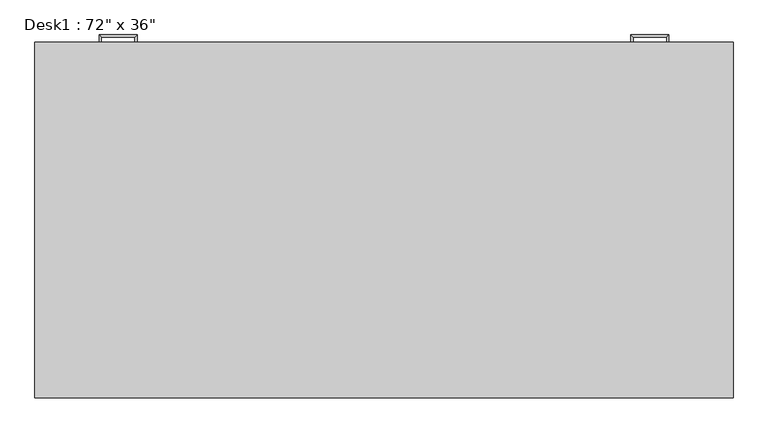
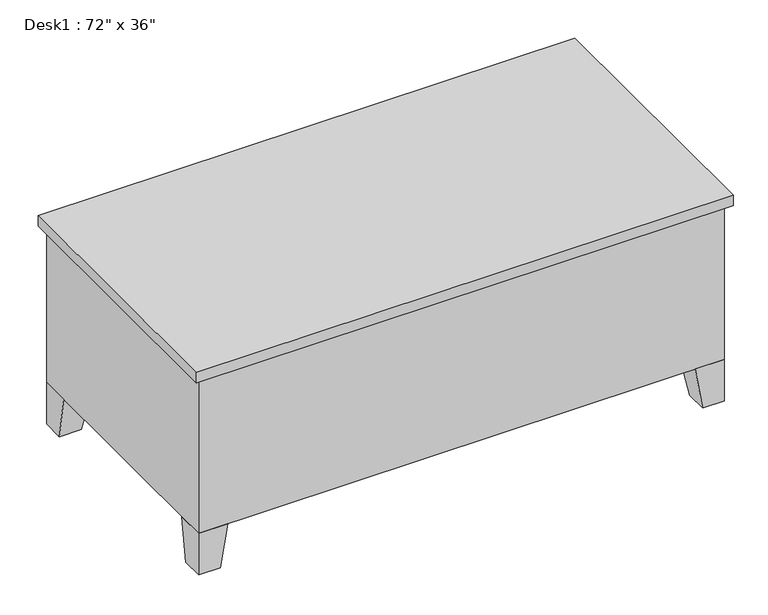
"""IFC4 building model written with IfcOpenShell, lengths in millimetres: furniture geometry."""

from ifc_helpers import new_model, si_unit, frame, origin, place, context, project, spatial, polyline, outline, extrude, faceted_brep, source, transform, mapped, element, save


def furniture_01cd08eb(model_context):
    return source(origin(), model_context, "Body", "SolidModel", [
        extrude(outline(polyline([(-133.35, 76.2), (-133.35, 88.9), (234.95, 88.9), (234.95, 76.2), (-133.35, 76.2)])), frame((0.0, 0.0, 603.25), z_axis=(0.0, 0.0, 1.0), x_axis=(1.0, 0.0, 0.0)), (0.0, 0.0, 1.0), 101.6),
        extrude(outline(polyline([(-133.35, 76.2), (-133.35, 88.9), (234.95, 88.9), (234.95, 76.2), (-133.35, 76.2)])), frame((0.0, 0.0, 171.45), z_axis=(0.0, 0.0, 1.0), x_axis=(1.0, 0.0, 0.0)), (0.0, 0.0, 1.0), 412.75),
        extrude(outline(polyline([(1289.05, 76.2), (1289.05, 88.9), (1657.35, 88.9), (1657.35, 76.2), (1289.05, 76.2)])), frame((0.0, 0.0, 603.25), z_axis=(0.0, 0.0, 1.0), x_axis=(1.0, 0.0, 0.0)), (0.0, 0.0, 1.0), 101.6),
        extrude(outline(polyline([(1289.05, 76.2), (1289.05, 88.9), (1657.35, 88.9), (1657.35, 76.2), (1289.05, 76.2)])), frame((0.0, 0.0, 171.45), z_axis=(0.0, 0.0, 1.0), x_axis=(1.0, 0.0, 0.0)), (0.0, 0.0, 1.0), 171.45),
        extrude(outline(polyline([(1289.05, 76.2), (1289.05, 88.9), (1657.35, 88.9), (1657.35, 76.2), (1289.05, 76.2)])), frame((0.0, 0.0, 482.6), z_axis=(0.0, 0.0, 1.0), x_axis=(1.0, 0.0, 0.0)), (0.0, 0.0, 1.0), 101.6),
        extrude(outline(polyline([(1289.05, 76.2), (1289.05, 88.9), (1657.35, 88.9), (1657.35, 76.2), (1289.05, 76.2)])), frame((0.0, 0.0, 361.95), z_axis=(0.0, 0.0, 1.0), x_axis=(1.0, 0.0, 0.0)), (0.0, 0.0, 1.0), 101.6),
        faceted_brep([(-50.8, 76.2, 152.4), (-152.4, 76.2, 152.4), (-152.4, -25.4, 152.4), (-50.8, -25.4, 152.4), (-76.2, 76.2, 0.0), (-76.2, 0.0, 0.0), (-152.4, 0.0, 0.0), (-152.4, 76.2, 0.0)], [[[0, 1, 2, 3]], [[4, 5, 6, 7]], [[4, 0, 3, 5]], [[5, 3, 2, 6]], [[6, 2, 1, 7]], [[7, 1, 0, 4]]]),
        faceted_brep([(-50.8, -838.2, 152.4), (-50.8, -736.6, 152.4), (-152.4, -736.6, 152.4), (-152.4, -838.2, 152.4), (-76.2, -838.2, 0.0), (-152.4, -838.2, 0.0), (-152.4, -762.0, 0.0), (-76.2, -762.0, 0.0)], [[[0, 1, 2, 3]], [[4, 5, 6, 7]], [[4, 0, 3, 5]], [[5, 3, 2, 6]], [[6, 2, 1, 7]], [[7, 1, 0, 4]]]),
        faceted_brep([(1574.8, -838.2, 152.4), (1676.4, -838.2, 152.4), (1676.4, -736.6, 152.4), (1574.8, -736.6, 152.4), (1600.2, -838.2, 0.0), (1600.2, -762.0, 0.0), (1676.4, -762.0, 0.0), (1676.4, -838.2, 0.0)], [[[0, 1, 2, 3]], [[4, 5, 6, 7]], [[4, 0, 3, 5]], [[5, 3, 2, 6]], [[6, 2, 1, 7]], [[7, 1, 0, 4]]]),
        faceted_brep([(1574.8, 76.2, 152.4), (1574.8, -25.4, 152.4), (1676.4, -25.4, 152.4), (1676.4, 76.2, 152.4), (1600.2, 76.2, 0.0), (1676.4, 76.2, 0.0), (1676.4, 0.0, 0.0), (1600.2, 0.0, 0.0)], [[[0, 1, 2, 3]], [[4, 5, 6, 7]], [[4, 0, 3, 5]], [[5, 3, 2, 6]], [[6, 2, 1, 7]], [[7, 1, 0, 4]]]),
        extrude(outline(polyline([(-171.45, 95.25), (1695.45, 95.25), (1695.45, -857.25), (-171.45, -857.25), (-171.45, 95.25)])), frame((0.0, 0.0, 723.9), z_axis=(0.0, 0.0, 1.0), x_axis=(1.0, 0.0, 0.0)), (0.0, 0.0, 1.0), 38.1),
        extrude(outline(polyline([(1270.0, 76.2), (1676.4, 76.2), (1676.4, -838.2), (-152.4, -838.2), (-152.4, 76.2), (254.0, 76.2), (254.0, -711.2), (1270.0, -711.2), (1270.0, 76.2)])), frame((0.0, 0.0, 152.4), z_axis=(0.0, 0.0, 1.0), x_axis=(1.0, 0.0, 0.0)), (0.0, 0.0, 1.0), 571.5),
        faceted_brep([(6.35, 88.9, 546.1), (0.0, 88.9, 546.1), (0.0, 88.9, 533.4), (6.35, 88.9, 533.4), (6.35, 107.95, 533.4), (6.35, 107.95, 546.1), (0.0, 114.3, 533.4), (0.0, 114.3, 546.1), (95.25, 107.95, 533.4), (95.25, 107.95, 546.1), (101.6, 114.3, 533.4), (101.6, 114.3, 546.1), (95.25, 88.9, 546.1), (95.25, 88.9, 533.4), (101.6, 88.9, 533.4), (101.6, 88.9, 546.1)], [[[0, 1, 2, 3]], [[3, 4, 5, 0]], [[2, 6, 4, 3]], [[1, 7, 6, 2]], [[0, 5, 7, 1]], [[4, 8, 9, 5]], [[6, 10, 8, 4]], [[7, 11, 10, 6]], [[5, 9, 11, 7]], [[12, 13, 14, 15]], [[8, 13, 12, 9]], [[10, 14, 13, 8]], [[11, 15, 14, 10]], [[9, 12, 15, 11]]]),
        faceted_brep([(6.35, 88.9, 666.75), (0.0, 88.9, 666.75), (0.0, 88.9, 654.05), (6.35, 88.9, 654.05), (6.35, 107.95, 654.05), (6.35, 107.95, 666.75), (0.0, 114.3, 654.05), (0.0, 114.3, 666.75), (95.25, 107.95, 654.05), (95.25, 107.95, 666.75), (101.6, 114.3, 654.05), (101.6, 114.3, 666.75), (95.25, 88.9, 666.75), (95.25, 88.9, 654.05), (101.6, 88.9, 654.05), (101.6, 88.9, 666.75)], [[[0, 1, 2, 3]], [[3, 4, 5, 0]], [[2, 6, 4, 3]], [[1, 7, 6, 2]], [[0, 5, 7, 1]], [[4, 8, 9, 5]], [[6, 10, 8, 4]], [[7, 11, 10, 6]], [[5, 9, 11, 7]], [[12, 13, 14, 15]], [[8, 13, 12, 9]], [[10, 14, 13, 8]], [[11, 15, 14, 10]], [[9, 12, 15, 11]]]),
        faceted_brep([(1517.65, 88.9, 304.8), (1517.65, 88.9, 292.1), (1524.0, 88.9, 292.1), (1524.0, 88.9, 304.8), (1524.0, 114.3, 304.8), (1517.65, 107.95, 304.8), (1524.0, 114.3, 292.1), (1517.65, 107.95, 292.1), (1422.4, 114.3, 304.8), (1428.75, 107.95, 304.8), (1422.4, 114.3, 292.1), (1428.75, 107.95, 292.1), (1428.75, 88.9, 304.8), (1422.4, 88.9, 304.8), (1422.4, 88.9, 292.1), (1428.75, 88.9, 292.1)], [[[0, 1, 2, 3]], [[3, 4, 5, 0]], [[2, 6, 4, 3]], [[1, 7, 6, 2]], [[0, 5, 7, 1]], [[4, 8, 9, 5]], [[6, 10, 8, 4]], [[7, 11, 10, 6]], [[5, 9, 11, 7]], [[12, 13, 14, 15]], [[8, 13, 12, 9]], [[10, 14, 13, 8]], [[11, 15, 14, 10]], [[9, 12, 15, 11]]]),
        faceted_brep([(1517.65, 88.9, 425.45), (1517.65, 88.9, 412.75), (1524.0, 88.9, 412.75), (1524.0, 88.9, 425.45), (1524.0, 114.3, 425.45), (1517.65, 107.95, 425.45), (1524.0, 114.3, 412.75), (1517.65, 107.95, 412.75), (1422.4, 114.3, 425.45), (1428.75, 107.95, 425.45), (1422.4, 114.3, 412.75), (1428.75, 107.95, 412.75), (1428.75, 88.9, 425.45), (1422.4, 88.9, 425.45), (1422.4, 88.9, 412.75), (1428.75, 88.9, 412.75)], [[[0, 1, 2, 3]], [[3, 4, 5, 0]], [[2, 6, 4, 3]], [[1, 7, 6, 2]], [[0, 5, 7, 1]], [[4, 8, 9, 5]], [[6, 10, 8, 4]], [[7, 11, 10, 6]], [[5, 9, 11, 7]], [[12, 13, 14, 15]], [[8, 13, 12, 9]], [[10, 14, 13, 8]], [[11, 15, 14, 10]], [[9, 12, 15, 11]]]),
        faceted_brep([(1517.65, 88.9, 546.1), (1517.65, 88.9, 533.4), (1524.0, 88.9, 533.4), (1524.0, 88.9, 546.1), (1524.0, 114.3, 546.1), (1517.65, 107.95, 546.1), (1524.0, 114.3, 533.4), (1517.65, 107.95, 533.4), (1422.4, 114.3, 546.1), (1428.75, 107.95, 546.1), (1422.4, 114.3, 533.4), (1428.75, 107.95, 533.4), (1428.75, 88.9, 546.1), (1422.4, 88.9, 546.1), (1422.4, 88.9, 533.4), (1428.75, 88.9, 533.4)], [[[0, 1, 2, 3]], [[3, 4, 5, 0]], [[2, 6, 4, 3]], [[1, 7, 6, 2]], [[0, 5, 7, 1]], [[4, 8, 9, 5]], [[6, 10, 8, 4]], [[7, 11, 10, 6]], [[5, 9, 11, 7]], [[12, 13, 14, 15]], [[8, 13, 12, 9]], [[10, 14, 13, 8]], [[11, 15, 14, 10]], [[9, 12, 15, 11]]]),
        faceted_brep([(1517.65, 88.9, 666.75), (1517.65, 88.9, 654.05), (1524.0, 88.9, 654.05), (1524.0, 88.9, 666.75), (1524.0, 114.3, 666.75), (1517.65, 107.95, 666.75), (1524.0, 114.3, 654.05), (1517.65, 107.95, 654.05), (1422.4, 114.3, 666.75), (1428.75, 107.95, 666.75), (1422.4, 114.3, 654.05), (1428.75, 107.95, 654.05), (1428.75, 88.9, 666.75), (1422.4, 88.9, 666.75), (1422.4, 88.9, 654.05), (1428.75, 88.9, 654.05)], [[[0, 1, 2, 3]], [[3, 4, 5, 0]], [[2, 6, 4, 3]], [[1, 7, 6, 2]], [[0, 5, 7, 1]], [[4, 8, 9, 5]], [[6, 10, 8, 4]], [[7, 11, 10, 6]], [[5, 9, 11, 7]], [[12, 13, 14, 15]], [[8, 13, 12, 9]], [[10, 14, 13, 8]], [[11, 15, 14, 10]], [[9, 12, 15, 11]]]),
    ])


if __name__ == "__main__":
    model = new_model("IFC4")
    model_context = context("Model", 3, world=origin())
    ifc_project = project(units=[si_unit("LENGTHUNIT", "METRE", prefix="MILLI")], contexts=[model_context])
    site = spatial("IfcSite", under=ifc_project)
    building = spatial("IfcBuilding", under=site)
    placement = place(None, origin())
    furniture_shape = furniture_01cd08eb(model_context)
    element("IfcFurniture", 1, ObjectType="Desk1 : 72\" x 36\"", at=placement, inside=building, context=model_context, shape_type="MappedRepresentation", body=[
        mapped(furniture_shape, transform((0.0, 0.0, 0.0), x_axis=(1.0, 0.0, 0.0), y_axis=(0.0, 1.0, 0.0), z_axis=(0.0, 0.0, 1.0))),
    ])
    save(model, "model.ifc")

# Revit data of these elements
# Type "Desk1 : 72\" x 36\""
#   Assembly Code = "E2020200"
#   Depth = 3' - 0"
#   Height = 2' - 6"
#   Leg Height = 0' - 6"
#   Width = 6' - 0"
#   Body Material = Laminate, Ivory, Matte
#   Handle/Leg Material = Steel, Chrome Plated
#   Top Material = Cherry
#   Default Elevation = 0
# Element 1 (IfcFurniture, "Desk1 : 72\" x 36\"")
#   Materials on its faces: "Steel, Chrome Plated", "Laminate, Ivory, Matte", "Cherry"
# Materials
#   "Laminate, Ivory, Matte": class "Plastic", colour RGB 247 247 239, transparency 0, Description = "Plastic Laminate - Ivory, Matte", Cost = 0
#   "Steel, Chrome Plated": class "Metal", colour RGB 17 17 17, transparency 0, Description = "Chromiuim plated steel", Cost = 0
#   "Cherry": class "Wood", colour RGB 226 177 128, transparency 0, Description = "Prunus Serotina", Cost = 0
